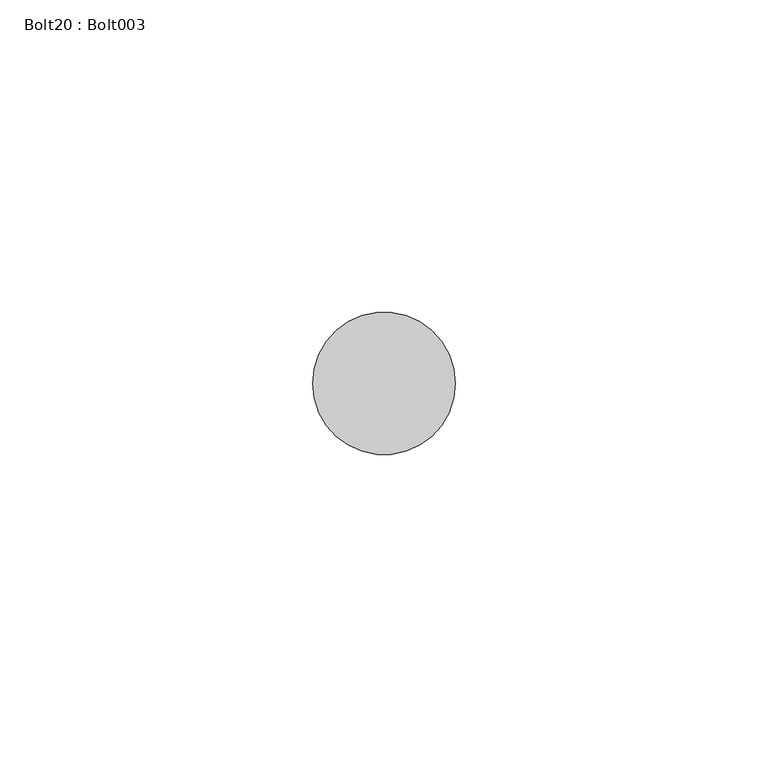
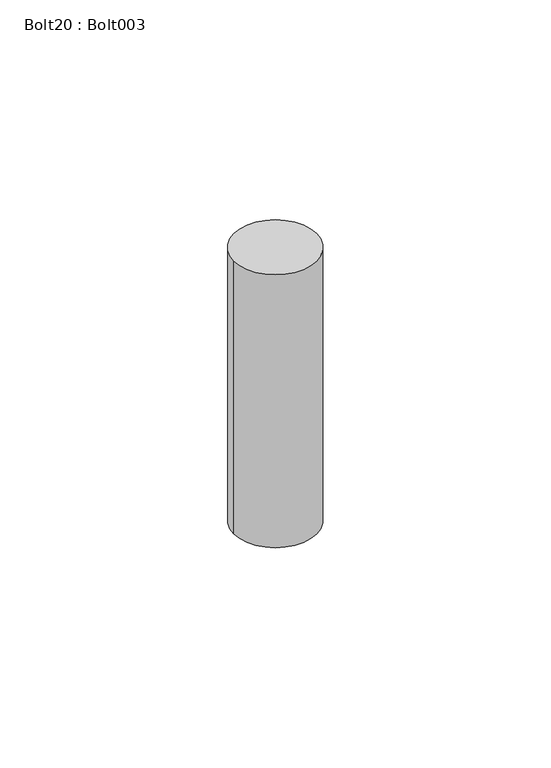
"""IFC4 building model written with IfcOpenShell, lengths in millimetres: proxy geometry, Bolt20 : Bolt003."""

from ifc_helpers import new_model, si_unit, point, frame, frame_2d, origin, place, context, project, spatial, circle_curve, trimmed, segment, composite_curve, outline, extrude, source, transform, mapped, element, save


def bolt20_bolt003_a01074e3(model_context):
    return source(origin(), model_context, "Body", "SweptSolid", [
        extrude(outline(composite_curve([segment(trimmed(circle_curve(frame_2d((7415.2612305, -1781.8449707)), 11.4045168), [point((7403.8567137, -1781.8449707))], [point((7426.6657473, -1781.8449707))], False, "CARTESIAN"), True, "CONTINUOUS"), segment(trimmed(circle_curve(frame_2d((7415.2612305, -1781.8449707)), 11.4045168), [point((7426.6657473, -1781.8449707))], [point((7403.8567137, -1781.8449707))], False, "CARTESIAN"), True, "CONTINUOUS")], self_intersect=False)), frame((0.0, 0.0, 40049.196), z_axis=(0.0, 0.0, 1.0), x_axis=(1.0, 0.0, 0.0)), (0.0, 0.0, 1.0), 79.375),
    ])


if __name__ == "__main__":
    model = new_model("IFC4")
    model_context = context("Model", 3, world=origin())
    ifc_project = project(units=[si_unit("LENGTHUNIT", "METRE", prefix="MILLI")], contexts=[model_context])
    site = spatial("IfcSite", under=ifc_project)
    building = spatial("IfcBuilding", under=site)
    placement = place(None, origin())
    bolt20_bolt003_shape = bolt20_bolt003_a01074e3(model_context)
    element("IfcBuildingElementProxy", 1, Name="Bolt20 : Bolt003", ObjectType="Bolt20 : Bolt003", at=placement, inside=building, context=model_context, shape_type="MappedRepresentation", body=[
        mapped(bolt20_bolt003_shape, transform((0.0, 0.0, 0.0), x_axis=(1.0, 0.0, 0.0), y_axis=(0.0, 1.0, 0.0), z_axis=(0.0, 0.0, 1.0))),
    ])
    save(model, "model.ifc")

# Revit data of these elements
# Type "Bolt20 : Bolt003"
#   NameOverride = "Bolt003"
# Element 1 (IfcBuildingElementProxy, "Bolt20 : Bolt003")
#   Materials on its faces: "BOLTS CONCEALED BY FLOOR FINISH"
# Materials
#   "BOLTS CONCEALED BY FLOOR FINISH": class "Unassigned", colour RGB 128 128 128, transparency 0
